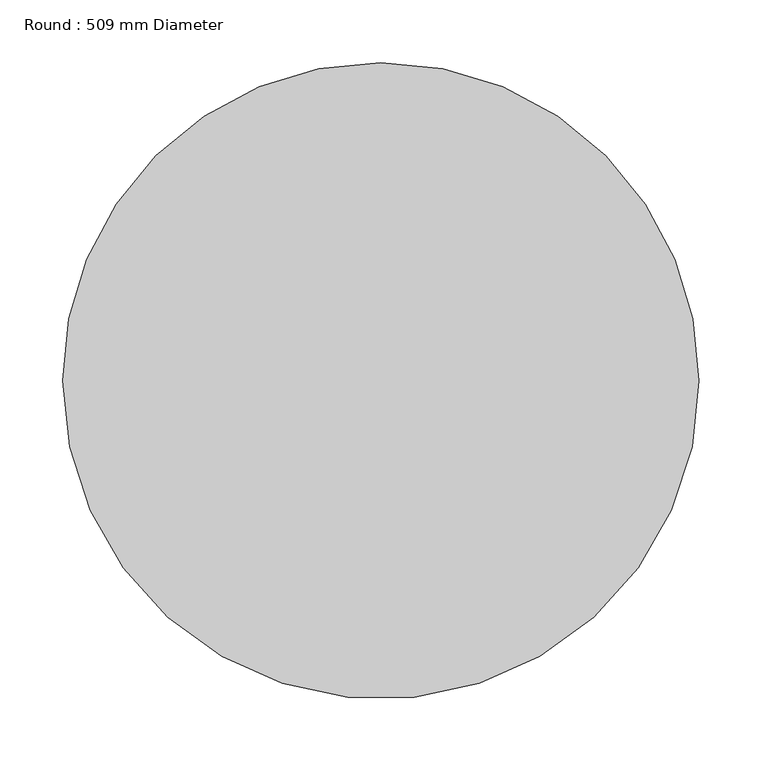
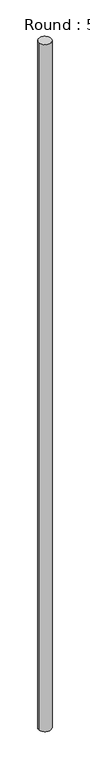
"""IFC4 building model written with IfcOpenShell, lengths in millimetres: column geometry, Round : 509 mm Diameter."""

from ifc_helpers import new_model, si_unit, point, frame, origin, origin_2d, place, context, project, spatial, circle_curve, trimmed, segment, composite_curve, outline, extrude, source, transform, mapped, element, save


def round_509_mm_diameter_8d8a8064(model_context):
    return source(origin(), model_context, "Body", "SweptSolid", [
        extrude(outline(composite_curve([segment(trimmed(circle_curve(origin_2d(), 254.0), [point((254.0, 0.0))], [point((-254.0, 0.0))], False, "CARTESIAN"), True, "CONTINUOUS"), segment(trimmed(circle_curve(origin_2d(), 254.0), [point((-254.0, 0.0))], [point((0.0, 254.0))], False, "CARTESIAN"), True, "CONTINUOUS"), segment(trimmed(circle_curve(origin_2d(), 254.0), [point((0.0, 254.0))], [point((254.0, 0.0))], False, "CARTESIAN"), True, "CONTINUOUS")], self_intersect=False)), frame((0.0, 0.0, 120100.0), z_axis=(0.0, 0.0, 1.0), x_axis=(1.0, 0.0, 0.0)), (0.0, 0.0, 1.0), 29281.4),
    ])


if __name__ == "__main__":
    model = new_model("IFC4")
    model_context = context("Model", 3, world=origin())
    ifc_project = project(units=[si_unit("LENGTHUNIT", "METRE", prefix="MILLI")], contexts=[model_context])
    site = spatial("IfcSite", under=ifc_project)
    building = spatial("IfcBuilding", under=site)
    placement = place(None, origin())
    round_509_mm_diameter_shape = round_509_mm_diameter_8d8a8064(model_context)
    element("IfcColumn", 1, ObjectType="Round : 509 mm Diameter", at=placement, inside=building, context=model_context, shape_type="MappedRepresentation", body=[
        mapped(round_509_mm_diameter_shape, transform((0.0, 0.0, 0.0), x_axis=(1.0, 0.0, 0.0), y_axis=(0.0, 1.0, 0.0), z_axis=(0.0, 0.0, 1.0))),
    ])
    save(model, "model.ifc")

# Revit data of these elements
# Type "Round : 509 mm Diameter"
#   Keynote = "G"
#   Diameter = 508.00 mm
#   Offset Base = 0.00 mm
#   Offset Top = 0.00 mm
#   built-in parameter 1002110 = 9474192
#   built-in parameter 1002106 = element 3
#   Material = Concrete - Cast In Situ
# Element 1 (IfcColumn, "Round : 509 mm Diameter")
#   Materials on its faces: "Concrete - Cast In Situ"
# Materials
#   "Concrete - Cast In Situ": class "Unassigned", colour RGB 255 255 255, transparency 0, Keynote = "E10/132", Cost = 0
